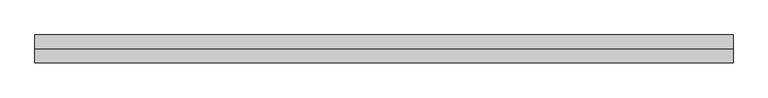
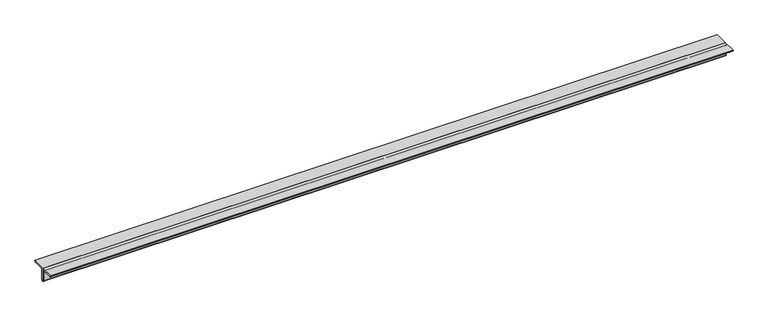
"""IFC4 building model written with IfcOpenShell, lengths in millimetres: member geometry, Steel Framing_2Ls_KS : H_SB_AR_S02_2Ls-100x100x10_VBR1."""

from ifc_helpers import new_model, si_unit, point, frame, frame_2d, origin, place, context, project, spatial, polyline, circle_curve, trimmed, segment, composite_curve, outline, extrude, source, transform, mapped, element, save


def member_4b2a810f(model_context):
    return source(origin(), model_context, "Body", "SweptSolid", [
        extrude(outline(composite_curve([segment(polyline([(0.0, 28.2), (100.0, 28.2)]), True, "CONTINUOUS"), segment(trimmed(circle_curve(frame_2d((90.0, 28.2)), 10.0), [point((100.0, 28.2))], [point((90.0, 18.2))], False, "CARTESIAN"), True, "CONTINUOUS"), segment(polyline([(90.0, 18.2), (20.0, 18.2)]), True, "CONTINUOUS"), segment(trimmed(circle_curve(frame_2d((20.0, 8.2)), 10.0), [point((20.0, 18.2))], [point((10.0, 8.2))], True, "CARTESIAN"), True, "CONTINUOUS"), segment(polyline([(10.0, 8.2), (10.0, -61.8)]), True, "CONTINUOUS"), segment(trimmed(circle_curve(frame_2d((0.0, -61.8)), 10.0), [point((10.0, -61.8))], [point((0.0, -71.8))], False, "CARTESIAN"), True, "CONTINUOUS"), segment(polyline([(0.0, -71.8), (0.0, 28.2)]), True, "CONTINUOUS")], self_intersect=False)), frame((-2444.561686, 0.0, 0.0), z_axis=(1.0, 0.0, 0.0), x_axis=(0.0, 1.0, 0.0)), (0.0, 0.0, 1.0), 5034.8971694),
        extrude(outline(composite_curve([segment(polyline([(0.0, 28.2), (0.0, -71.8)]), True, "CONTINUOUS"), segment(trimmed(circle_curve(frame_2d((0.0, -61.8)), 10.0), [point((0.0, -71.8))], [point((-10.0, -61.8))], False, "CARTESIAN"), True, "CONTINUOUS"), segment(polyline([(-10.0, -61.8), (-10.0, 8.2)]), True, "CONTINUOUS"), segment(trimmed(circle_curve(frame_2d((-20.0, 8.2)), 10.0), [point((-10.0, 8.2))], [point((-20.0, 18.2))], True, "CARTESIAN"), True, "CONTINUOUS"), segment(polyline([(-20.0, 18.2), (-90.0, 18.2)]), True, "CONTINUOUS"), segment(trimmed(circle_curve(frame_2d((-90.0, 28.2)), 10.0), [point((-90.0, 18.2))], [point((-100.0, 28.2))], False, "CARTESIAN"), True, "CONTINUOUS"), segment(polyline([(-100.0, 28.2), (0.0, 28.2)]), True, "CONTINUOUS")], self_intersect=False)), frame((-2444.561686, 0.0, 0.0), z_axis=(1.0, 0.0, 0.0), x_axis=(0.0, 1.0, 0.0)), (0.0, 0.0, 1.0), 5034.8971694),
    ])


if __name__ == "__main__":
    model = new_model("IFC4")
    model_context = context("Model", 3, world=origin())
    ifc_project = project(units=[si_unit("LENGTHUNIT", "METRE", prefix="MILLI")], contexts=[model_context])
    site = spatial("IfcSite", under=ifc_project)
    building = spatial("IfcBuilding", under=site)
    placement = place(None, origin())
    member_shape = member_4b2a810f(model_context)
    element("IfcMember", 1, ObjectType="Steel Framing_2Ls_KS : H_SB_AR_S02_2Ls-100x100x10_VBR1", at=placement, inside=building, context=model_context, shape_type="MappedRepresentation", body=[
        mapped(member_shape, transform((0.0, 0.0, 0.0), x_axis=(1.0, 0.0, 0.0), y_axis=(0.0, 1.0, 0.0), z_axis=(0.0, 0.0, 1.0))),
    ])
    save(model, "model.ifc")

# Revit data of these elements
# Type "Steel Framing_2Ls_KS : H_SB_AR_S02_2Ls-100x100x10_VBR1"
#   Type Comments = "MAIN"
#   Type Mark = "VBR1"
#   H_SectionID = "2Ls-100x100x10"
#   Assembly Code = "B10"
#   Legs = "LLBB"
#   H_Ratio for Additional Steel Plate = 0.2
#   W = 0
#   Perimeter = 0.80 m²/m
#   Nominal Weight = 29.80 kgf/m
#   Length [instance default] = 1524 mm
#   Space = 0 mm
#   b = 100 mm
#   d = 100 mm
#   t = 10 mm
#   y = 28.2 mm
#   A = 0.0038 m²
#   Structural Material [instance default] = Steel, 45-345
# Element 1 (IfcMember, "Steel Framing_2Ls_KS : H_SB_AR_S02_2Ls-100x100x10_VBR1")
#   Materials on its faces: "Steel, 45-345"
# Materials
#   "Steel, 45-345": class "Metal", colour RGB 189 187 185, transparency 0, Description = "Steel 345 MPa", Cost = 0
